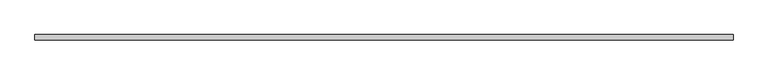
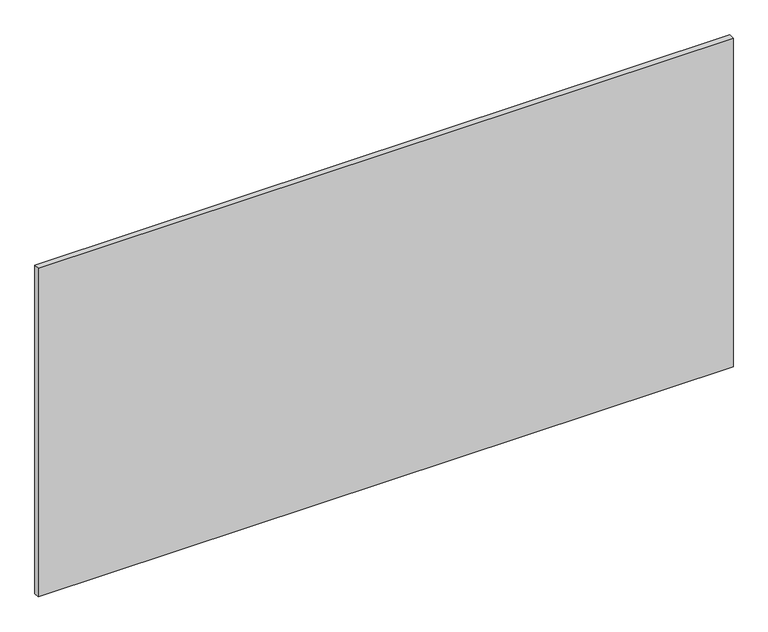
"""IFC4 building model written with IfcOpenShell, lengths in millimetres: proxy geometry, Inner panel:Inner panel:1:Inner panel:1 : Inner panel:Inner panel:300324:300043:Inner panel:1:Inner panel:1 : Inner panel:Inner panel:300324:300043 : Inner panel:Inner panel:1:Inner panel:1 : Inner panel:Inner panel:300324:300043:22 : Inner panel:Inner panel:1:Inner panel:1 : Inner panel:Inner panel:300324:300043:Inner panel:1:Inner panel:1 : Inner panel:Inner panel:300324:300043 : Inner panel:Inner panel:1:Inner panel:1 : Inner panel:Inner panel:300324:300043:300031."""

import ifcopenshell
import ifcopenshell.guid

model = None  # the IFC model being written
_history = None  # IfcOwnerHistory: only IFC2X3 demands one
_inside = {}  # id of a spatial element -> (the spatial element, [elements in it])
_under = {}  # id of a project, library or spatial element -> (it, [spatial elements below it])
_declared = {}  # id of a project -> (the project, [libraries it declares])
_typed = {}  # id of a type object -> (the type object, [elements of that type])
_made_of = {}  # id of a material, layer set ... -> (it, [elements and type objects made of it])


def new_model(schema):
    """Start an empty IFC model of exactly this schema.

    Asked for "IFC4X3", IfcOpenShell would pick the latest addendum, in which some entities
    have other attributes; the version numbers below select the first issue.
    IFC2X3 requires an IfcOwnerHistory on every rooted entity: one is made here for all.
    """
    global model, _history
    if schema == "IFC4X3":
        model = ifcopenshell.file(schema_version=(4, 3, 0, 0))
    else:
        model = ifcopenshell.file(schema=schema)
    _inside.clear()
    _under.clear()
    _declared.clear()
    _typed.clear()
    _made_of.clear()
    _history = None
    if model.schema == "IFC2X3":
        org = make("IfcOrganization", Name="unknown")
        user = make(
            "IfcPersonAndOrganization",
            ThePerson=make("IfcPerson", FamilyName="unknown"),
            TheOrganization=org,
        )
        app = make(
            "IfcApplication",
            ApplicationDeveloper=org,
            Version="unknown",
            ApplicationFullName="unknown",
            ApplicationIdentifier="unknown",
        )
        _history = make(
            "IfcOwnerHistory",
            OwningUser=user,
            OwningApplication=app,
            ChangeAction="ADDED",
            CreationDate=0,
        )
    return model


def make(cls, **values):
    """One entity of the class cls with the attributes given. An attribute that is None is left unset."""
    return model.create_entity(
        cls, **{name: value for name, value in values.items() if value is not None}
    )


def rooted(cls, **values):
    """An entity with a GlobalId (a new one), such as an element, a storey or a relation."""
    return make(cls, GlobalId=ifcopenshell.guid.new(), OwnerHistory=_history, **values)


def si_unit(unit_type, name, prefix=None):
    """IfcSIUnit, for example si_unit("LENGTHUNIT", "METRE", prefix="MILLI")."""
    return make("IfcSIUnit", UnitType=unit_type, Prefix=prefix, Name=name)


def assignment(units):
    """IfcUnitAssignment: the units of a project."""
    return None if units is None else make("IfcUnitAssignment", Units=units)


def point(xyz):
    """IfcCartesianPoint."""
    return None if xyz is None else make("IfcCartesianPoint", Coordinates=xyz)


def direction(xyz):
    """IfcDirection."""
    return None if xyz is None else make("IfcDirection", DirectionRatios=xyz)


def frame(location, z_axis=None, x_axis=None):
    """IfcAxis2Placement3D, a coordinate frame: its origin and axes. An axis left out is left unset."""
    return make(
        "IfcAxis2Placement3D",
        Location=point(location),
        Axis=direction(z_axis),
        RefDirection=direction(x_axis),
    )


def origin():
    """The frame at (0, 0, 0) with its axes left unset."""
    return frame((0.0, 0.0, 0.0))


def place(relative_to, where):
    """IfcLocalPlacement: puts the frame where relative to a parent placement (None: the world)."""
    return make(
        "IfcLocalPlacement", PlacementRelTo=relative_to, RelativePlacement=where
    )


def context(
    kind, dimensions, precision=None, world=None, true_north=None, identifier=None
):
    """IfcGeometricRepresentationContext, for example the 3D "Model" context."""
    return make(
        "IfcGeometricRepresentationContext",
        ContextIdentifier=identifier,
        ContextType=kind,
        CoordinateSpaceDimension=dimensions,
        Precision=precision,
        WorldCoordinateSystem=world,
        TrueNorth=true_north,
    )


def project(units=None, contexts=None):
    """IfcProject with its units and contexts."""
    return rooted(
        "IfcProject",
        Name="project",
        RepresentationContexts=contexts,
        UnitsInContext=assignment(units),
    )


def spatial(cls, under=None, at=None, **own):
    """A site, building, storey or space (cls), placed at a placement, below another one or the project."""
    s = rooted(cls, ObjectPlacement=at, **own)
    if under is not None:
        _under.setdefault(under.id(), (under, []))[1].append(s)
    return s


def polyline(points):
    """IfcPolyline through the points."""
    return make("IfcPolyline", Points=[point(p) for p in points])


def outline(outer, holes=None, kind="AREA"):
    """IfcArbitraryClosedProfileDef: a profile drawn as a closed curve; with holes, ...WithVoids."""
    if holes is None:
        return make("IfcArbitraryClosedProfileDef", ProfileType=kind, OuterCurve=outer)
    return make(
        "IfcArbitraryProfileDefWithVoids",
        ProfileType=kind,
        OuterCurve=outer,
        InnerCurves=holes,
    )


def extrude(swept, where, along, depth):
    """IfcExtrudedAreaSolid: the profile swept, set in the frame where, extruded along a direction by depth."""
    return make(
        "IfcExtrudedAreaSolid",
        SweptArea=swept,
        Position=where,
        ExtrudedDirection=direction(along),
        Depth=depth,
    )


def shape(context_of_items, identifier, shape_type, items):
    """IfcShapeRepresentation: the items that make up one representation, for example the "Body"."""
    return make(
        "IfcShapeRepresentation",
        ContextOfItems=context_of_items,
        RepresentationIdentifier=identifier,
        RepresentationType=shape_type,
        Items=items,
    )


def source(mapping_origin, context_of_items, identifier, shape_type, items):
    """IfcRepresentationMap: a shape defined once, which mapped items show again and again."""
    return make(
        "IfcRepresentationMap",
        MappingOrigin=mapping_origin,
        MappedRepresentation=shape(context_of_items, identifier, shape_type, items),
    )


def transform(
    local_origin,
    x_axis=None,
    y_axis=None,
    z_axis=None,
    scale=None,
    scale2=None,
    scale3=None,
    uniform=True,
):
    """IfcCartesianTransformationOperator3D, or its non-uniform kind. x_axis, y_axis, z_axis: its Axis1, 2, 3."""
    if uniform:
        return make(
            "IfcCartesianTransformationOperator3D",
            Axis1=direction(x_axis),
            Axis2=direction(y_axis),
            LocalOrigin=point(local_origin),
            Scale=scale,
            Axis3=direction(z_axis),
        )
    return make(
        "IfcCartesianTransformationOperator3DnonUniform",
        Axis1=direction(x_axis),
        Axis2=direction(y_axis),
        LocalOrigin=point(local_origin),
        Scale=scale,
        Axis3=direction(z_axis),
        Scale2=scale2,
        Scale3=scale3,
    )


def mapped(mapping_source, mapping_target):
    """IfcMappedItem: shows the shape of a source again, moved by a transform."""
    return make(
        "IfcMappedItem", MappingSource=mapping_source, MappingTarget=mapping_target
    )


def made_of(thing, what):
    """Note that an element or type object is made of a material, layer set ...; save() writes the relation."""
    if what is not None:
        _made_of.setdefault(what.id(), (what, []))[1].append(thing)
    return thing


def element(
    cls,
    number,
    at=None,
    inside=None,
    cuts=None,
    type_object=None,
    material=None,
    context=None,
    identifier="Body",
    shape_type=None,
    held_by="IfcProductDefinitionShape",
    body=None,
    shapes=None,
    **own,
):
    """One element of the class cls, such as IfcWall. Its Tag is "e" and its number.

    at: its placement. inside: the storey or other place that contains it. cuts: it is an
    opening in that element (IfcRelVoidsElement). A single representation is given by context,
    identifier, shape_type and body (its items); several are given by shapes. held_by: the class
    of the entity that holds the representations. save() writes the other relations.
    """
    e = rooted(cls, Tag="e%d" % number, ObjectPlacement=at, **own)
    if body is not None:
        shapes = [shape(context, identifier, shape_type, body)]
    if shapes is not None:
        e.Representation = make(held_by, Representations=shapes)
    if inside is not None:
        _inside.setdefault(inside.id(), (inside, []))[1].append(e)
    if cuts is not None:
        rooted(
            "IfcRelVoidsElement", RelatingBuildingElement=cuts, RelatedOpeningElement=e
        )
    if type_object is not None:
        _typed.setdefault(type_object.id(), (type_object, []))[1].append(e)
    return made_of(e, material)


def aggregate(whole, parts):
    """IfcRelAggregates: a whole, such as a stair, and the parts it consists of."""
    return rooted("IfcRelAggregates", RelatingObject=whole, RelatedObjects=parts)


def save(model, path):
    """Write the relations noted so far, then the file.

    IfcRelAggregates (storeys below a building ...), IfcRelContainedInSpatialStructure (elements
    in a storey), IfcRelDefinesByType, IfcRelAssociatesMaterial and IfcRelDeclares: one each for
    every whole, place, type object, material and project.
    """
    for whole, parts in _under.values():
        aggregate(whole, parts)
    for where, things in _inside.values():
        rooted(
            "IfcRelContainedInSpatialStructure",
            RelatedElements=things,
            RelatingStructure=where,
        )
    for kind, things in _typed.values():
        rooted("IfcRelDefinesByType", RelatedObjects=things, RelatingType=kind)
    for what, things in _made_of.values():
        rooted("IfcRelAssociatesMaterial", RelatedObjects=things, RelatingMaterial=what)
    for by, libraries in _declared.values():
        rooted("IfcRelDeclares", RelatingContext=by, RelatedDefinitions=libraries)
    model.write(path)


def generic_models_5df29abb(model_context):
    return source(origin(), model_context, "Body", "SweptSolid", [
        extrude(outline(polyline([(593738.0867239, -567913.5913841), (596176.4867239, -567913.5913841), (596176.4867239, -567932.6413841), (593738.0867239, -567932.6413841), (593738.0867239, -567913.5913841)])), frame((0.0, 0.0, 2495.55), z_axis=(0.0, 0.0, 1.0), x_axis=(1.0, 0.0, 0.0)), (0.0, 0.0, 1.0), 1219.2),
    ])


if __name__ == "__main__":
    model = new_model("IFC4")
    model_context = context("Model", 3, world=origin())
    ifc_project = project(units=[si_unit("LENGTHUNIT", "METRE", prefix="MILLI")], contexts=[model_context])
    site = spatial("IfcSite", under=ifc_project)
    building = spatial("IfcBuilding", under=site)
    placement = place(None, origin())
    generic_models_shape = generic_models_5df29abb(model_context)
    element("IfcBuildingElementProxy", 1, Name="Inner panel:Inner panel:1:Inner panel:1 : Inner panel:Inner panel:300324:300043:Inner panel:1:Inner panel:1 : Inner panel:Inner panel:300324:300043 : Inner panel:Inner panel:1:Inner panel:1 : Inner panel:Inner panel:300324:300043:22 : Inner panel:Inner panel:1:Inner panel:1 : Inner panel:Inner panel:300324:300043:Inner panel:1:Inner panel:1 : Inner panel:Inner panel:300324:300043 : Inner panel:Inner panel:1:Inner panel:1 : Inner panel:Inner panel:300324:300043:300031", ObjectType="Inner panel:Inner panel:1:Inner panel:1 : Inner panel:Inner panel:300324:300043:Inner panel:1:Inner panel:1 : Inner panel:Inner panel:300324:300043 : Inner panel:Inner panel:1:Inner panel:1 : Inner panel:Inner panel:300324:300043:22 : Inner panel:Inner panel:1:Inner panel:1 : Inner panel:Inner panel:300324:300043:Inner panel:1:Inner panel:1 : Inner panel:Inner panel:300324:300043 : Inner panel:Inner panel:1:Inner panel:1 : Inner panel:Inner panel:300324:300043:300031", at=placement, inside=building, context=model_context, shape_type="MappedRepresentation", body=[
        mapped(generic_models_shape, transform((0.0, 0.0, 0.0), x_axis=(1.0, 0.0, 0.0), y_axis=(0.0, 1.0, 0.0), z_axis=(0.0, 0.0, 1.0))),
    ])
    save(model, "model.ifc")

# Revit data of these elements
# Type "Inner panel:Inner panel:1:Inner panel:1 : Inner panel:Inner panel:300324:300043:Inner panel:1:Inner panel:1 : Inner panel:Inner panel:300324:300043 : Inner panel:Inner panel:1:Inner panel:1 : Inner panel:Inner panel:300324:300043:22 : Inner panel:Inner panel:1:Inner panel:1 : Inner panel:Inner panel:300324:300043:Inner panel:1:Inner panel:1 : Inner panel:Inner panel:300324:300043 : Inner panel:Inner panel:1:Inner panel:1 : Inner panel:Inner panel:300324:300043:300031"
#   NameOverride = "Inner panel:Inner panel:1:Inner panel:1 : Inner panel:Inner panel:300324:300043:Inner panel:1:Inner panel:1 : Inner panel:Inner panel:300324:300043 : Inner panel:Inner panel:1:Inner panel:1 : Inner panel:Inner panel:300324:300043:300031"
#   ObjectTypeOverride = "Inner panel:1:Inner panel:1 : Inner panel:Inner panel:300324:300043 : Inner panel:Inner panel:1:Inner panel:1 : Inner panel:Inner panel:300324:300043"
#   Reference = "Inner panel"
#   Tag = "300031"
# Element 1 (IfcBuildingElementProxy, "Inner panel:Inner panel:1:Inner panel:1 : Inner panel:Inner panel:300324:300043:Inner panel:1:Inner panel:1 : Inner panel:Inner panel:300324:300043 : Inner panel:Inner panel:1:Inner panel:1 : Inner panel:Inner panel:300324:300043:22 : Inner panel:Inner panel:1:Inner panel:1 : Inner panel:Inner panel:300324:300043:Inner panel:1:Inner panel:1 : Inner panel:Inner panel:300324:300043 : Inner panel:Inner panel:1:Inner panel:1 : Inner panel:Inner panel:300324:300043:300031")
#   Materials on its faces: "¾” (CLASS A) FIRE RETARDANT PLYWOOD ...OR… IF 1/4\" GYP. BD UNDER PLYWOOD, FLAME SPREAD TO BE CLASS C -  (FINISH: GRADE B - PREFINISHED STAINED/SEALED) - 1/4\" GAP BTWN PANELS (FASTENERS T.B.D.)"
# Materials
#   "¾” (CLASS A) FIRE RETARDANT PLYWOOD ...OR… IF 1/4\" GYP. BD UNDER PLYWOOD, FLAME SPREAD TO BE CLASS C -  (FINISH: GRADE B - PREFINISHED STAINED/SEALED) - 1/4\" GAP BTWN PANELS (FASTENERS T.B.D.)": class "Wood", colour RGB 149 120 74, transparency 0, Description = "Plywood, sheathing grade", Cost = 0
